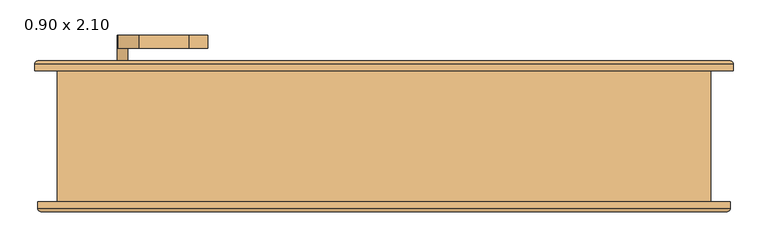
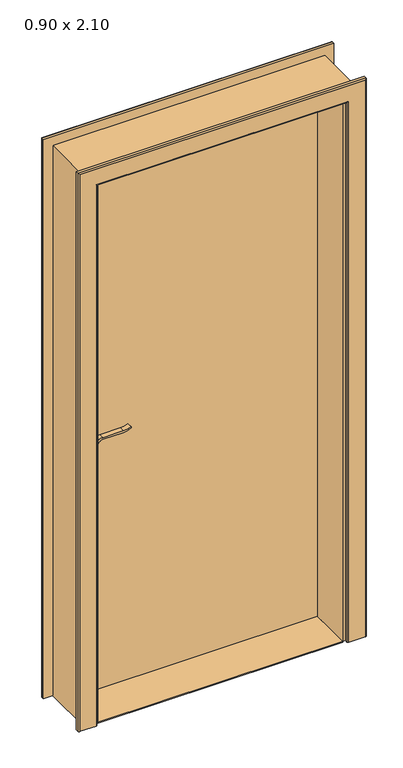
"""IFC4 building model written with IfcOpenShell, lengths in millimetres: door geometry, PORTA_DE_ABRIR_MADEIRA : 0.90 x 2.10."""

from ifc_helpers import new_model, si_unit, point, frame, frame_2d, origin, origin_with_axes, place, context, project, spatial, polyline, circle_curve, ellipse_curve, trimmed, segment, composite_curve, outline, extrude, faceted_brep, source, transform, mapped, element, save
from ifc_brep_helpers import plane_surface, cylinder_surface, advanced_brep


def door_0_90_x_2_10_c767737c(model_context):
    return source(origin(), model_context, "Body", "SolidModel", [
        extrude(outline(composite_curve([segment(trimmed(circle_curve(frame_2d((940.0, -400.0)), 15.0), [point((940.0, -385.0))], [point((940.0, -415.0))], False, "CARTESIAN"), True, "CONTINUOUS"), segment(trimmed(circle_curve(frame_2d((940.0, -400.0)), 15.0), [point((940.0, -415.0))], [point((940.0, -385.0))], False, "CARTESIAN"), True, "CONTINUOUS")], self_intersect=False)), frame((0.0, 40.0, 0.0), z_axis=(0.0, 1.0, 0.0), x_axis=(0.0, 0.0, 1.0)), (0.0, 0.0, 1.0), 10.0),
        extrude(outline(composite_curve([segment(trimmed(circle_curve(frame_2d((940.0, -400.0)), 15.0), [point((940.0, -385.0))], [point((940.0, -415.0))], False, "CARTESIAN"), True, "CONTINUOUS"), segment(trimmed(circle_curve(frame_2d((940.0, -400.0)), 15.0), [point((940.0, -415.0))], [point((940.0, -385.0))], False, "CARTESIAN"), True, "CONTINUOUS")], self_intersect=False)), frame((0.0, 105.0, 0.0), z_axis=(0.0, 1.0, 0.0), x_axis=(0.0, 0.0, 1.0)), (0.0, 0.0, 1.0), 10.0),
        extrude(outline(composite_curve([segment(trimmed(circle_curve(frame_2d((1000.0, -400.0)), 8.0), [point((1004.6523287, -406.5081363))], [point((1000.0, -392.0))], False, "CARTESIAN"), True, "CONTINUOUS"), segment(trimmed(circle_curve(frame_2d((994.8738613, -374.6138099)), 18.1261387), [point((1000.0, -392.0))], [point((1013.0, -374.6138099))], True, "CARTESIAN"), True, "CONTINUOUS"), segment(polyline([(1013.0, -374.6138099), (1013.0, -298.3564091)]), True, "CONTINUOUS"), segment(trimmed(circle_curve(frame_2d((1072.2709207, -301.9396612)), 59.3791355), [point((1013.0, -298.3564091))], [point((1022.2135558, -270.0))], False, "CARTESIAN"), True, "CONTINUOUS"), segment(polyline([(1022.2135558, -270.0), (1025.0, -270.0)]), True, "CONTINUOUS"), segment(trimmed(circle_curve(frame_2d((1103.2850638, -298.4227909)), 83.2850902), [point((1025.0, -270.0))], [point((1020.0, -298.3564091))], True, "CARTESIAN"), True, "CONTINUOUS"), segment(polyline([(1020.0, -298.3564091), (1020.0, -374.6325667)]), True, "CONTINUOUS"), segment(trimmed(circle_curve(frame_2d((982.7555521, -376.3324871)), 37.2832219), [point((1020.0, -374.6325667))], [point((1004.6523287, -406.5081363))], False, "CARTESIAN"), True, "CONTINUOUS")], self_intersect=False)), frame((0.0, 0.0, 0.0), z_axis=(0.0, 1.0, 0.0), x_axis=(0.0, 0.0, 1.0)), (0.0, 0.0, 1.0), 20.0),
        extrude(outline(composite_curve([segment(trimmed(circle_curve(frame_2d((994.8738682, -374.6138122)), 18.1261318), [point((999.9999903, -392.0))], [point((1013.0, -374.6138122))], True, "CARTESIAN"), True, "CONTINUOUS"), segment(polyline([(1013.0, -374.6138122), (1013.0, -298.3564091)]), True, "CONTINUOUS"), segment(trimmed(circle_curve(frame_2d((1072.2709207, -301.9396612)), 59.3791355), [point((1013.0, -298.3564091))], [point((1022.2135558, -270.0))], False, "CARTESIAN"), True, "CONTINUOUS"), segment(polyline([(1022.2135558, -270.0), (1025.0, -270.0)]), True, "CONTINUOUS"), segment(trimmed(circle_curve(frame_2d((1103.2850638, -298.4227909)), 83.2850902), [point((1025.0, -270.0))], [point((1020.0, -298.3564091))], True, "CARTESIAN"), True, "CONTINUOUS"), segment(polyline([(1020.0, -298.3564091), (1020.0, -374.6325667)]), True, "CONTINUOUS"), segment(trimmed(circle_curve(frame_2d((982.7555521, -376.3324871)), 37.2832219), [point((1020.0, -374.6325667))], [point((1004.6523287, -406.5081363))], False, "CARTESIAN"), True, "CONTINUOUS"), segment(trimmed(circle_curve(frame_2d((1000.0, -400.0)), 8.0), [point((1004.6523287, -406.5081363))], [point((999.9999903, -392.0))], False, "CARTESIAN"), True, "CONTINUOUS")], self_intersect=False)), frame((0.0, 135.0, 0.0), z_axis=(0.0, 1.0, 0.0), x_axis=(0.0, 0.0, 1.0)), (0.0, 0.0, 1.0), 20.0),
        extrude(outline(composite_curve([segment(trimmed(circle_curve(frame_2d((1000.0, -400.0)), 8.0), [point((1000.0, -392.0))], [point((1000.0, -408.0))], False, "CARTESIAN"), True, "CONTINUOUS"), segment(trimmed(circle_curve(frame_2d((1000.0, -400.0)), 8.0), [point((1000.0, -408.0))], [point((1000.0, -392.0))], False, "CARTESIAN"), True, "CONTINUOUS")], self_intersect=False)), frame((0.0, 20.0, 0.0), z_axis=(0.0, 1.0, 0.0), x_axis=(0.0, 0.0, 1.0)), (0.0, 0.0, 1.0), 30.0),
        extrude(outline(composite_curve([segment(trimmed(circle_curve(frame_2d((1000.0, -400.0)), 8.0), [point((1000.0, -392.0))], [point((1000.0, -408.0))], False, "CARTESIAN"), True, "CONTINUOUS"), segment(trimmed(circle_curve(frame_2d((1000.0, -400.0)), 8.0), [point((1000.0, -408.0))], [point((1000.0, -392.0))], False, "CARTESIAN"), True, "CONTINUOUS")], self_intersect=False)), frame((0.0, 105.0, 0.0), z_axis=(0.0, 1.0, 0.0), x_axis=(0.0, 0.0, 1.0)), (0.0, 0.0, 1.0), 30.0),
        extrude(outline(composite_curve([segment(trimmed(circle_curve(frame_2d((930.0, -400.0)), 25.0), [point((930.0, -425.0))], [point((930.0, -375.0))], False, "CARTESIAN"), True, "CONTINUOUS"), segment(polyline([(930.0, -375.0), (1000.0, -375.0)]), True, "CONTINUOUS"), segment(trimmed(circle_curve(frame_2d((1000.0, -400.0)), 25.0), [point((1000.0, -375.0))], [point((1000.0, -425.0))], False, "CARTESIAN"), True, "CONTINUOUS"), segment(polyline([(1000.0, -425.0), (930.0, -425.0)]), True, "CONTINUOUS")], self_intersect=False)), frame((0.0, 50.0, 0.0), z_axis=(0.0, 1.0, 0.0), x_axis=(0.0, 0.0, 1.0)), (0.0, 0.0, 1.0), 10.0),
        extrude(outline(composite_curve([segment(trimmed(circle_curve(frame_2d((930.0, -400.0)), 25.0), [point((930.0, -425.0))], [point((930.0, -375.0))], False, "CARTESIAN"), True, "CONTINUOUS"), segment(polyline([(930.0, -375.0), (1000.0, -375.0)]), True, "CONTINUOUS"), segment(trimmed(circle_curve(frame_2d((1000.0, -400.0)), 25.0), [point((1000.0, -375.0))], [point((1000.0, -425.0))], False, "CARTESIAN"), True, "CONTINUOUS"), segment(polyline([(1000.0, -425.0), (930.0, -425.0)]), True, "CONTINUOUS")], self_intersect=False)), frame((0.0, 95.0, 0.0), z_axis=(0.0, 1.0, 0.0), x_axis=(0.0, 0.0, 1.0)), (0.0, 0.0, 1.0), 10.0),
        faceted_brep([(-460.0, 60.0, 0.0), (-450.0, 60.0, 0.0), (-450.0, -100.0, 0.0), (-500.0, -100.0, 0.0), (-500.0, 100.0, 0.0), (-460.0, 100.0, 0.0), (-460.0, 100.0, 2100.0), (-460.0, 60.0, 2100.0), (-500.0, 100.0, 2140.0), (500.0, 100.0, 2140.0), (500.0, 100.0, 0.0), (460.0, 100.0, 0.0), (460.0, 100.0, 2100.0), (-500.0, -100.0, 2140.0), (-450.0, -100.0, 2090.0), (450.0, -100.0, 2090.0), (450.0, -100.0, 0.0), (500.0, -100.0, 0.0), (500.0, -100.0, 2140.0), (-450.0, 60.0, 2090.0), (460.0, 60.0, 2100.0), (460.0, 60.0, 0.0), (450.0, 60.0, 0.0), (450.0, 60.0, 2090.0)], [[[0, 1, 2, 3, 4, 5]], [[5, 6, 7, 0]], [[4, 8, 9, 10, 11, 12, 6, 5]], [[3, 13, 8, 4]], [[2, 14, 15, 16, 17, 18, 13, 3]], [[1, 19, 14, 2]], [[0, 7, 20, 21, 22, 23, 19, 1]], [[23, 22, 16, 15]], [[21, 11, 10, 17, 16, 22]], [[12, 11, 21, 20]], [[18, 17, 10, 9]], [[13, 18, 9, 8]], [[19, 23, 15, 14]], [[6, 12, 20, 7]]]),
        advanced_brep(
        [(-530.0, -100.3, 0.0), (-460.0, -100.3, 0.0), (-460.0, -110.3, 0.0), (-465.0, -115.3, 0.0), (-525.0, -115.3, 0.0), (-530.0, -110.3, 0.0), (-530.0, -110.3, 2170.0), (-530.0, -100.3, 2170.0), (-525.0, -115.3, 2165.0), (-465.0, -115.3, 2105.0), (465.0, -115.3, 2105.0), (465.0, -115.3, 0.0), (525.0, -115.3, 0.0), (525.0, -115.3, 2165.0), (-460.0, -110.3, 2100.0), (-460.0, -100.3, 2100.0), (530.0, -100.3, 2170.0), (530.0, -100.3, 0.0), (460.0, -100.3, 0.0), (460.0, -100.3, 2100.0), (530.0, -110.3, 0.0), (460.0, -110.3, 0.0), (460.0, -110.3, 2100.0), (530.0, -110.3, 2170.0)],
        [
            (0, 1),
            (1, 2),
            (2, 3, circle_curve(frame((-465.0, -110.3, 0.0), z_axis=(0.0, 0.0, -1.0), x_axis=(-1.0, 0.0, 0.0)), 5.0)),
            (3, 4),
            (4, 5, circle_curve(frame((-525.0, -110.3, 0.0), z_axis=(0.0, 0.0, -1.0), x_axis=(-1.0, 0.0, 0.0)), 5.0)),
            (5, 0),
            (5, 6),
            (6, 7),
            (7, 0),
            (4, 8),
            (8, 6, ellipse_curve(frame((-525.0, -110.3, 2165.0), z_axis=(-0.7071067811865475, 0.0, -0.7071067811865475), x_axis=(0.7071067811865474, 0.0, -0.7071067811865476)), 7.0710678, 5.0)),
            (3, 9),
            (9, 10),
            (10, 11),
            (11, 12),
            (12, 13),
            (13, 8),
            (2, 14),
            (14, 9, ellipse_curve(frame((-465.0, -110.3, 2105.0), z_axis=(-0.7071067811865475, 0.0, -0.7071067811865475), x_axis=(0.7071067811865474, 0.0, -0.7071067811865476)), 7.0710678, 5.0)),
            (1, 15),
            (15, 14),
            (7, 16),
            (16, 17),
            (17, 18),
            (18, 19),
            (19, 15),
            (17, 20),
            (20, 12, circle_curve(frame((525.0, -110.3, 0.0), z_axis=(0.0, 0.0, -1.0), x_axis=(1.0, 0.0, 0.0)), 5.0)),
            (11, 21, circle_curve(frame((465.0, -110.3, 0.0), z_axis=(0.0, 0.0, -1.0), x_axis=(1.0, 0.0, 0.0)), 5.0)),
            (21, 18),
            (21, 22),
            (22, 19),
            (10, 22, ellipse_curve(frame((465.0, -110.3, 2105.0), z_axis=(0.7071067811865475, 0.0, -0.7071067811865475), x_axis=(0.7071067811865474, 0.0, 0.7071067811865476)), 7.0710678, 5.0)),
            (20, 23),
            (23, 13, ellipse_curve(frame((525.0, -110.3, 2165.0), z_axis=(0.7071067811865475, 0.0, -0.7071067811865475), x_axis=(0.7071067811865474, 0.0, 0.7071067811865476)), 7.0710678, 5.0)),
            (16, 23),
            (6, 23),
            (22, 14),
        ],
        [
            plane_surface(frame((-500.0, 100.0, 0.0), z_axis=(0.0, 0.0, -1.0), x_axis=(0.0, 1.0, 0.0))),
            plane_surface(frame((-530.0, -100.3, 0.0), z_axis=(-1.0, 0.0, 0.0), x_axis=(0.0, 0.0, 1.0))),
            cylinder_surface(frame((-525.0, -110.3, 0.0), z_axis=(0.0, 0.0, -1.0), x_axis=(-1.0, 0.0, 0.0)), 5.0),
            plane_surface(frame((-525.0, -115.3, 0.0), z_axis=(0.0, -1.0, 0.0), x_axis=(0.0, 0.0, 1.0))),
            cylinder_surface(frame((-465.0, -110.3, 0.0), z_axis=(0.0, 0.0, -1.0), x_axis=(-1.0, 0.0, 0.0)), 5.0),
            plane_surface(frame((-460.0, -110.3, 0.0), z_axis=(1.0, 0.0, 0.0), x_axis=(0.0, 0.0, 1.0))),
            plane_surface(frame((-460.0, -100.3, 0.0), z_axis=(0.0, 1.0, 0.0), x_axis=(0.0, 0.0, 1.0))),
            plane_surface(frame((500.0, 100.0, 0.0), z_axis=(0.0, 0.0, -1.0), x_axis=(0.0, 1.0, 0.0))),
            plane_surface(frame((460.0, -110.3, 2100.0), z_axis=(-1.0, 0.0, 0.0), x_axis=(0.0, 0.0, -1.0))),
            cylinder_surface(frame((465.0, -110.3, 2140.0), z_axis=(0.0, 0.0, 1.0), x_axis=(1.0, 0.0, 0.0)), 5.0),
            cylinder_surface(frame((525.0, -110.3, 2140.0), z_axis=(0.0, 0.0, 1.0), x_axis=(1.0, 0.0, 0.0)), 5.0),
            plane_surface(frame((530.0, -100.3, 2170.0), z_axis=(1.0, 0.0, 0.0), x_axis=(0.0, 0.0, -1.0))),
            plane_surface(frame((-530.0, -100.3, 2170.0), z_axis=(0.0, 0.0, 1.0), x_axis=(1.0, 0.0, 0.0))),
            plane_surface(frame((-460.0, -110.3, 2100.0), z_axis=(0.0, 0.0, -1.0), x_axis=(1.0, 0.0, 0.0))),
            cylinder_surface(frame((-500.0, -110.3, 2165.0), z_axis=(-1.0, 0.0, 0.0), x_axis=(0.0, 0.0, 1.0)), 5.0),
            cylinder_surface(frame((-500.0, -110.3, 2105.0), z_axis=(-1.0, 0.0, 0.0), x_axis=(0.0, 0.0, 1.0)), 5.0),
        ],
        [
            (0, [[1, 2, 3, 4, 5, 6]]),
            (1, [[7, 8, 9, -6]]),
            (2, [[10, 11, -7, -5]]),
            (3, [[12, 13, 14, 15, 16, 17, -10, -4]]),
            (4, [[18, 19, -12, -3]]),
            (5, [[20, 21, -18, -2]]),
            (6, [[-9, 22, 23, 24, 25, 26, -20, -1]]),
            (7, [[27, 28, -15, 29, 30, -24]]),
            (8, [[-25, -30, 31, 32]]),
            (9, [[-31, -29, -14, 33]]),
            (10, [[-16, -28, 34, 35]]),
            (11, [[-34, -27, -23, 36]]),
            (12, [[37, -36, -22, -8]]),
            (13, [[-26, -32, 38, -21]]),
            (14, [[-17, -35, -37, -11]]),
            (15, [[-38, -33, -13, -19]]),
        ],
    ),
        advanced_brep(
        [(-529.3155593, 115.2647517, 0.0), (-469.3155593, 115.2647517, 0.0), (-464.3155593, 110.2647517, 0.0), (-464.3155593, 100.2647517, 0.0), (-534.3155593, 100.2647517, 0.0), (-534.3155593, 110.2647517, 0.0), (-534.3155593, 110.2647517, 2174.3155593), (-529.3155593, 115.2647517, 2169.3155593), (-534.3155593, 100.2647517, 2174.3155593), (-464.3155593, 100.2647517, 2104.3155593), (464.3155593, 100.2647517, 2104.3155593), (464.3155593, 100.2647517, 0.0), (534.3155593, 100.2647517, 0.0), (534.3155593, 100.2647517, 2174.3155593), (-464.3155593, 110.2647517, 2104.3155593), (-469.3155593, 115.2647517, 2109.3155593), (529.3155593, 115.2647517, 2169.3155593), (529.3155593, 115.2647517, 0.0), (469.3155593, 115.2647517, 0.0), (469.3155593, 115.2647517, 2109.3155593), (534.3155593, 110.2647517, 0.0), (464.3155593, 110.2647517, 0.0), (464.3155593, 110.2647517, 2104.3155593), (534.3155593, 110.2647517, 2174.3155593)],
        [
            (0, 1),
            (1, 2, circle_curve(frame((-469.3155593, 110.2647517, 0.0), z_axis=(0.0, 0.0, -1.0), x_axis=(-1.0, 0.0, 0.0)), 5.0)),
            (2, 3),
            (3, 4),
            (4, 5),
            (5, 0, circle_curve(frame((-529.3155593, 110.2647517, 0.0), z_axis=(0.0, 0.0, -1.0), x_axis=(-1.0, 0.0, 0.0)), 5.0)),
            (5, 6),
            (6, 7, ellipse_curve(frame((-529.3155593, 110.2647517, 2169.3155593), z_axis=(-0.7071067811865475, 0.0, -0.7071067811865475), x_axis=(0.7071067811865474, 0.0, -0.7071067811865476)), 7.0710678, 5.0)),
            (7, 0),
            (4, 8),
            (8, 6),
            (3, 9),
            (9, 10),
            (10, 11),
            (11, 12),
            (12, 13),
            (13, 8),
            (2, 14),
            (14, 9),
            (1, 15),
            (15, 14, ellipse_curve(frame((-469.3155593, 110.2647517, 2109.3155593), z_axis=(-0.7071067811865475, 0.0, -0.7071067811865475), x_axis=(0.7071067811865474, 0.0, -0.7071067811865476)), 7.0710678, 5.0)),
            (7, 16),
            (16, 17),
            (17, 18),
            (18, 19),
            (19, 15),
            (17, 20, circle_curve(frame((529.3155593, 110.2647517, 0.0), z_axis=(0.0, 0.0, -1.0), x_axis=(1.0, 0.0, 0.0)), 5.0)),
            (20, 12),
            (11, 21),
            (21, 18, circle_curve(frame((469.3155593, 110.2647517, 0.0), z_axis=(0.0, 0.0, -1.0), x_axis=(1.0, 0.0, 0.0)), 5.0)),
            (21, 22),
            (22, 19, ellipse_curve(frame((469.3155593, 110.2647517, 2109.3155593), z_axis=(0.7071067811865475, 0.0, -0.7071067811865475), x_axis=(0.7071067811865474, 0.0, 0.7071067811865476)), 7.0710678, 5.0)),
            (10, 22),
            (20, 23),
            (23, 13),
            (16, 23, ellipse_curve(frame((529.3155593, 110.2647517, 2169.3155593), z_axis=(0.7071067811865475, 0.0, -0.7071067811865475), x_axis=(0.7071067811865474, 0.0, 0.7071067811865476)), 7.0710678, 5.0)),
            (23, 6),
            (14, 22),
        ],
        [
            plane_surface(frame((-500.0, 100.0, 0.0), z_axis=(0.0, 0.0, -1.0), x_axis=(0.0, 1.0, 0.0))),
            cylinder_surface(frame((-529.3155593, 110.2647517, 0.0), z_axis=(0.0, 0.0, -1.0), x_axis=(-1.0, 0.0, 0.0)), 5.0),
            plane_surface(frame((-534.3155593, 110.2647517, 0.0), z_axis=(-1.0, 0.0, 0.0), x_axis=(0.0, 0.0, 1.0))),
            plane_surface(frame((-534.3155593, 100.2647517, 0.0), z_axis=(0.0, -1.0, 0.0), x_axis=(0.0, 0.0, 1.0))),
            plane_surface(frame((-464.3155593, 100.2647517, 0.0), z_axis=(1.0, 0.0, 0.0), x_axis=(0.0, 0.0, 1.0))),
            cylinder_surface(frame((-469.3155593, 110.2647517, 0.0), z_axis=(0.0, 0.0, -1.0), x_axis=(-1.0, 0.0, 0.0)), 5.0),
            plane_surface(frame((-469.3155593, 115.2647517, 0.0), z_axis=(0.0, 1.0, 0.0), x_axis=(0.0, 0.0, 1.0))),
            plane_surface(frame((500.0, 100.0, 0.0), z_axis=(0.0, 0.0, -1.0), x_axis=(0.0, 1.0, 0.0))),
            cylinder_surface(frame((469.3155593, 110.2647517, 2140.0), z_axis=(0.0, 0.0, 1.0), x_axis=(1.0, 0.0, 0.0)), 5.0),
            plane_surface(frame((464.3155593, 100.2647517, 2104.3155593), z_axis=(-1.0, 0.0, 0.0), x_axis=(0.0, 0.0, -1.0))),
            plane_surface(frame((534.3155593, 110.2647517, 2174.3155593), z_axis=(1.0, 0.0, 0.0), x_axis=(0.0, 0.0, -1.0))),
            cylinder_surface(frame((529.3155593, 110.2647517, 2140.0), z_axis=(0.0, 0.0, 1.0), x_axis=(1.0, 0.0, 0.0)), 5.0),
            plane_surface(frame((-534.3155593, 110.2647517, 2174.3155593), z_axis=(0.0, 0.0, 1.0), x_axis=(1.0, 0.0, 0.0))),
            plane_surface(frame((-464.3155593, 100.2647517, 2104.3155593), z_axis=(0.0, 0.0, -1.0), x_axis=(1.0, 0.0, 0.0))),
            cylinder_surface(frame((-500.0, 110.2647517, 2169.3155593), z_axis=(-1.0, 0.0, 0.0), x_axis=(0.0, 0.0, 1.0)), 5.0),
            cylinder_surface(frame((-500.0, 110.2647517, 2109.3155593), z_axis=(-1.0, 0.0, 0.0), x_axis=(0.0, 0.0, 1.0)), 5.0),
        ],
        [
            (0, [[1, 2, 3, 4, 5, 6]]),
            (1, [[7, 8, 9, -6]]),
            (2, [[10, 11, -7, -5]]),
            (3, [[12, 13, 14, 15, 16, 17, -10, -4]]),
            (4, [[18, 19, -12, -3]]),
            (5, [[20, 21, -18, -2]]),
            (6, [[-9, 22, 23, 24, 25, 26, -20, -1]]),
            (7, [[27, 28, -15, 29, 30, -24]]),
            (8, [[-25, -30, 31, 32]]),
            (9, [[-31, -29, -14, 33]]),
            (10, [[-16, -28, 34, 35]]),
            (11, [[-34, -27, -23, 36]]),
            (12, [[-17, -35, 37, -11]]),
            (13, [[38, -33, -13, -19]]),
            (14, [[-37, -36, -22, -8]]),
            (15, [[-26, -32, -38, -21]]),
        ],
    ),
        extrude(outline(polyline([(460.0, 95.0), (460.0, 60.0), (-460.0, 60.0), (-460.0, 95.0), (460.0, 95.0)])), origin_with_axes(), (0.0, 0.0, 1.0), 2100.0),
        extrude(outline(polyline([(-450.0, 35.0), (-460.0, 35.0), (-460.0, 100.0), (460.0, 100.0), (460.0, 35.0), (450.0, 35.0), (450.0, -100.0), (-450.0, -100.0), (-450.0, 35.0)])), frame((0.0, 0.0, -3.0), z_axis=(0.0, 0.0, 1.0), x_axis=(1.0, 0.0, 0.0)), (0.0, 0.0, 1.0), 3.1),
    ])


if __name__ == "__main__":
    model = new_model("IFC4")
    model_context = context("Model", 3, world=origin())
    ifc_project = project(units=[si_unit("LENGTHUNIT", "METRE", prefix="MILLI")], contexts=[model_context])
    site = spatial("IfcSite", under=ifc_project)
    building = spatial("IfcBuilding", under=site)
    placement = place(None, origin())
    door_0_90_x_2_10_shape = door_0_90_x_2_10_c767737c(model_context)
    element("IfcDoor", 1, ObjectType="PORTA_DE_ABRIR_MADEIRA : 0.90 x 2.10", at=placement, inside=building, context=model_context, shape_type="MappedRepresentation", body=[
        mapped(door_0_90_x_2_10_shape, transform((0.0, 0.0, 0.0), x_axis=(1.0, 0.0, 0.0), y_axis=(0.0, 1.0, 0.0), z_axis=(0.0, 0.0, 1.0))),
    ])
    save(model, "model.ifc")

# Revit data of these elements
# Type "PORTA_DE_ABRIR_MADEIRA : 0.90 x 2.10"
#   Type Mark = "P1"
#   Analytic Construction = "<Nenhum>"
#   Rough Width = 1.00 m
#   Projeção da estrutura externa = 0.50 m
#   Projeção da estrutura interna = 0.025 m
#   Largura da estrutura = 0.075 m
#   Rough Height = 2.15 m
#   Height = 2.10 m
#   Width = 0.90 m
#   Soleira [instance default] = no
#   Material do batente = .BATENTE E GUARNIÇÃO
#   Material da maçaneta = .AÇO INOXIDÁVEL ESCOVADO
#   Material da folha da porta = .FOLHA DA PORTA
#   Material da Soleira [instance default] = none
#   Function = (empty or 0)
#   Wall Closure = (empty or 0)
# Element 1 (IfcDoor, "PORTA_DE_ABRIR_MADEIRA : 0.90 x 2.10")
#   Soleira = yes
#   Material da Soleira = .GRANITO BRANCO ITAUNAS
#   Materials on its faces: ".AÇO INOXIDÁVEL ESCOVADO", ".BATENTE E GUARNIÇÃO", ".GRANITO BRANCO ITAUNAS", ".FOLHA DA PORTA"
# Materials
#   ".BATENTE E GUARNIÇÃO": class "Madeira", colour RGB 215 186 156, transparency 0, Cost = 0
#   ".AÇO INOXIDÁVEL ESCOVADO": class "Metal", colour RGB 189 187 185, transparency 0, Description = "Stainless Steel 18/8, brushed finish", Cost = 0
#   ".FOLHA DA PORTA": class "Madeira", colour RGB 148 119 91, transparency 0, Cost = 0
#   ".GRANITO BRANCO ITAUNAS": class ".CC_PEDRA REVEST.", colour RGB 202 195 174, transparency 0, Description = "Revestimento em granito", Cost = 0
